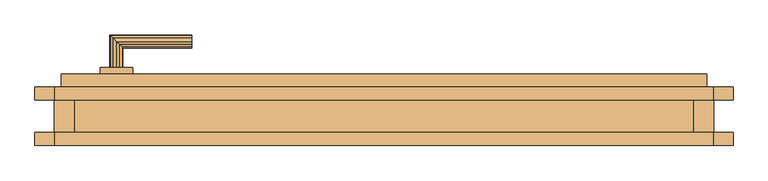
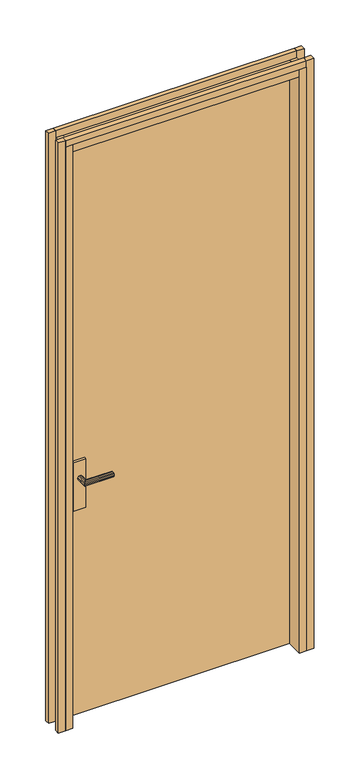
"""IFC4 building model written with IfcOpenShell, lengths in millimetres: door geometry, Tür."""

import ifcopenshell
import ifcopenshell.guid

model = None  # the IFC model being written
_history = None  # IfcOwnerHistory: only IFC2X3 demands one
_inside = {}  # id of a spatial element -> (the spatial element, [elements in it])
_under = {}  # id of a project, library or spatial element -> (it, [spatial elements below it])
_declared = {}  # id of a project -> (the project, [libraries it declares])
_typed = {}  # id of a type object -> (the type object, [elements of that type])
_made_of = {}  # id of a material, layer set ... -> (it, [elements and type objects made of it])


def new_model(schema):
    """Start an empty IFC model of exactly this schema.

    Asked for "IFC4X3", IfcOpenShell would pick the latest addendum, in which some entities
    have other attributes; the version numbers below select the first issue.
    IFC2X3 requires an IfcOwnerHistory on every rooted entity: one is made here for all.
    """
    global model, _history
    if schema == "IFC4X3":
        model = ifcopenshell.file(schema_version=(4, 3, 0, 0))
    else:
        model = ifcopenshell.file(schema=schema)
    _inside.clear()
    _under.clear()
    _declared.clear()
    _typed.clear()
    _made_of.clear()
    _history = None
    if model.schema == "IFC2X3":
        org = make("IfcOrganization", Name="unknown")
        user = make(
            "IfcPersonAndOrganization",
            ThePerson=make("IfcPerson", FamilyName="unknown"),
            TheOrganization=org,
        )
        app = make(
            "IfcApplication",
            ApplicationDeveloper=org,
            Version="unknown",
            ApplicationFullName="unknown",
            ApplicationIdentifier="unknown",
        )
        _history = make(
            "IfcOwnerHistory",
            OwningUser=user,
            OwningApplication=app,
            ChangeAction="ADDED",
            CreationDate=0,
        )
    return model


def make(cls, **values):
    """One entity of the class cls with the attributes given. An attribute that is None is left unset."""
    return model.create_entity(
        cls, **{name: value for name, value in values.items() if value is not None}
    )


def rooted(cls, **values):
    """An entity with a GlobalId (a new one), such as an element, a storey or a relation."""
    return make(cls, GlobalId=ifcopenshell.guid.new(), OwnerHistory=_history, **values)


def si_unit(unit_type, name, prefix=None):
    """IfcSIUnit, for example si_unit("LENGTHUNIT", "METRE", prefix="MILLI")."""
    return make("IfcSIUnit", UnitType=unit_type, Prefix=prefix, Name=name)


def assignment(units):
    """IfcUnitAssignment: the units of a project."""
    return None if units is None else make("IfcUnitAssignment", Units=units)


def point(xyz):
    """IfcCartesianPoint."""
    return None if xyz is None else make("IfcCartesianPoint", Coordinates=xyz)


def direction(xyz):
    """IfcDirection."""
    return None if xyz is None else make("IfcDirection", DirectionRatios=xyz)


def frame(location, z_axis=None, x_axis=None):
    """IfcAxis2Placement3D, a coordinate frame: its origin and axes. An axis left out is left unset."""
    return make(
        "IfcAxis2Placement3D",
        Location=point(location),
        Axis=direction(z_axis),
        RefDirection=direction(x_axis),
    )


def origin():
    """The frame at (0, 0, 0) with its axes left unset."""
    return frame((0.0, 0.0, 0.0))


def place(relative_to, where):
    """IfcLocalPlacement: puts the frame where relative to a parent placement (None: the world)."""
    return make(
        "IfcLocalPlacement", PlacementRelTo=relative_to, RelativePlacement=where
    )


def context(
    kind, dimensions, precision=None, world=None, true_north=None, identifier=None
):
    """IfcGeometricRepresentationContext, for example the 3D "Model" context."""
    return make(
        "IfcGeometricRepresentationContext",
        ContextIdentifier=identifier,
        ContextType=kind,
        CoordinateSpaceDimension=dimensions,
        Precision=precision,
        WorldCoordinateSystem=world,
        TrueNorth=true_north,
    )


def project(units=None, contexts=None):
    """IfcProject with its units and contexts."""
    return rooted(
        "IfcProject",
        Name="project",
        RepresentationContexts=contexts,
        UnitsInContext=assignment(units),
    )


def spatial(cls, under=None, at=None, **own):
    """A site, building, storey or space (cls), placed at a placement, below another one or the project."""
    s = rooted(cls, ObjectPlacement=at, **own)
    if under is not None:
        _under.setdefault(under.id(), (under, []))[1].append(s)
    return s


def polyline(points):
    """IfcPolyline through the points."""
    return make("IfcPolyline", Points=[point(p) for p in points])


def outline(outer, holes=None, kind="AREA"):
    """IfcArbitraryClosedProfileDef: a profile drawn as a closed curve; with holes, ...WithVoids."""
    if holes is None:
        return make("IfcArbitraryClosedProfileDef", ProfileType=kind, OuterCurve=outer)
    return make(
        "IfcArbitraryProfileDefWithVoids",
        ProfileType=kind,
        OuterCurve=outer,
        InnerCurves=holes,
    )


def extrude(swept, where, along, depth):
    """IfcExtrudedAreaSolid: the profile swept, set in the frame where, extruded along a direction by depth."""
    return make(
        "IfcExtrudedAreaSolid",
        SweptArea=swept,
        Position=where,
        ExtrudedDirection=direction(along),
        Depth=depth,
    )


def faces_of(points, faces, orient=None, outer=None):
    """IfcFace entities. A face is a list of loops; a loop is a list of indices into points, from 0.

    orient and outer hold one flag for each loop. By default every Orientation is true, the
    first loop of a face is its IfcFaceOuterBound and the others are IfcFaceBound.
    """
    made = []
    for i, loops in enumerate(faces):
        bounds = []
        for j, loop in enumerate(loops):
            is_outer = j == 0 if outer is None else outer[i][j]
            bounds.append(
                make(
                    "IfcFaceOuterBound" if is_outer else "IfcFaceBound",
                    Bound=make("IfcPolyLoop", Polygon=[points[k] for k in loop]),
                    Orientation=True if orient is None else orient[i][j],
                )
            )
        made.append(make("IfcFace", Bounds=bounds))
    return made


def faceted_brep(points, faces, orient=None, outer=None, voids=None):
    """IfcFacetedBrep: a solid bounded by flat faces; with voids (closed shells), ...WithVoids."""
    shared = [point(p) for p in points]
    hull = make("IfcClosedShell", CfsFaces=faces_of(shared, faces, orient, outer))
    if voids is None:
        return make("IfcFacetedBrep", Outer=hull)
    return make(
        "IfcFacetedBrepWithVoids",
        Outer=hull,
        Voids=[
            make(cls, CfsFaces=faces_of(shared, fs, o, b)) for cls, fs, o, b in voids
        ],
    )


def shape(context_of_items, identifier, shape_type, items):
    """IfcShapeRepresentation: the items that make up one representation, for example the "Body"."""
    return make(
        "IfcShapeRepresentation",
        ContextOfItems=context_of_items,
        RepresentationIdentifier=identifier,
        RepresentationType=shape_type,
        Items=items,
    )


def source(mapping_origin, context_of_items, identifier, shape_type, items):
    """IfcRepresentationMap: a shape defined once, which mapped items show again and again."""
    return make(
        "IfcRepresentationMap",
        MappingOrigin=mapping_origin,
        MappedRepresentation=shape(context_of_items, identifier, shape_type, items),
    )


def transform(
    local_origin,
    x_axis=None,
    y_axis=None,
    z_axis=None,
    scale=None,
    scale2=None,
    scale3=None,
    uniform=True,
):
    """IfcCartesianTransformationOperator3D, or its non-uniform kind. x_axis, y_axis, z_axis: its Axis1, 2, 3."""
    if uniform:
        return make(
            "IfcCartesianTransformationOperator3D",
            Axis1=direction(x_axis),
            Axis2=direction(y_axis),
            LocalOrigin=point(local_origin),
            Scale=scale,
            Axis3=direction(z_axis),
        )
    return make(
        "IfcCartesianTransformationOperator3DnonUniform",
        Axis1=direction(x_axis),
        Axis2=direction(y_axis),
        LocalOrigin=point(local_origin),
        Scale=scale,
        Axis3=direction(z_axis),
        Scale2=scale2,
        Scale3=scale3,
    )


def mapped(mapping_source, mapping_target):
    """IfcMappedItem: shows the shape of a source again, moved by a transform."""
    return make(
        "IfcMappedItem", MappingSource=mapping_source, MappingTarget=mapping_target
    )


def made_of(thing, what):
    """Note that an element or type object is made of a material, layer set ...; save() writes the relation."""
    if what is not None:
        _made_of.setdefault(what.id(), (what, []))[1].append(thing)
    return thing


def element(
    cls,
    number,
    at=None,
    inside=None,
    cuts=None,
    type_object=None,
    material=None,
    context=None,
    identifier="Body",
    shape_type=None,
    held_by="IfcProductDefinitionShape",
    body=None,
    shapes=None,
    **own,
):
    """One element of the class cls, such as IfcWall. Its Tag is "e" and its number.

    at: its placement. inside: the storey or other place that contains it. cuts: it is an
    opening in that element (IfcRelVoidsElement). A single representation is given by context,
    identifier, shape_type and body (its items); several are given by shapes. held_by: the class
    of the entity that holds the representations. save() writes the other relations.
    """
    e = rooted(cls, Tag="e%d" % number, ObjectPlacement=at, **own)
    if body is not None:
        shapes = [shape(context, identifier, shape_type, body)]
    if shapes is not None:
        e.Representation = make(held_by, Representations=shapes)
    if inside is not None:
        _inside.setdefault(inside.id(), (inside, []))[1].append(e)
    if cuts is not None:
        rooted(
            "IfcRelVoidsElement", RelatingBuildingElement=cuts, RelatedOpeningElement=e
        )
    if type_object is not None:
        _typed.setdefault(type_object.id(), (type_object, []))[1].append(e)
    return made_of(e, material)


def aggregate(whole, parts):
    """IfcRelAggregates: a whole, such as a stair, and the parts it consists of."""
    return rooted("IfcRelAggregates", RelatingObject=whole, RelatedObjects=parts)


def save(model, path):
    """Write the relations noted so far, then the file.

    IfcRelAggregates (storeys below a building ...), IfcRelContainedInSpatialStructure (elements
    in a storey), IfcRelDefinesByType, IfcRelAssociatesMaterial and IfcRelDeclares: one each for
    every whole, place, type object, material and project.
    """
    for whole, parts in _under.values():
        aggregate(whole, parts)
    for where, things in _inside.values():
        rooted(
            "IfcRelContainedInSpatialStructure",
            RelatedElements=things,
            RelatingStructure=where,
        )
    for kind, things in _typed.values():
        rooted("IfcRelDefinesByType", RelatedObjects=things, RelatingType=kind)
    for what, things in _made_of.values():
        rooted("IfcRelAssociatesMaterial", RelatedObjects=things, RelatingMaterial=what)
    for by, libraries in _declared.values():
        rooted("IfcRelDeclares", RelatingContext=by, RelatedDefinitions=libraries)
    model.write(path)


def door_23b21fe2(model_context):
    return source(origin(), model_context, "Body", "SolidModel", [
        faceted_brep([(100.0, 100.0, 1198.660254), (95.0, 100.0, 1200.0), (90.0, 100.0, 1198.660254), (86.339746, 100.0, 1195.0), (85.0, 100.0, 1190.0), (86.339746, 100.0, 1185.0), (90.0, 100.0, 1181.339746), (95.0, 100.0, 1180.0), (100.0, 100.0, 1181.339746), (103.660254, 100.0, 1185.0), (105.0, 100.0, 1190.0), (103.660254, 100.0, 1195.0), (95.0, 140.0, 1200.0), (90.0, 145.0, 1198.660254), (86.339746, 148.660254, 1195.0), (85.0, 150.0, 1190.0), (86.339746, 148.660254, 1185.0), (90.0, 145.0, 1181.339746), (95.0, 140.0, 1180.0), (100.0, 135.0, 1181.339746), (103.660254, 131.339746, 1185.0), (105.0, 130.0, 1190.0), (103.660254, 131.339746, 1195.0), (100.0, 135.0, 1198.660254), (210.0, 145.0, 1198.660254), (210.0, 140.0, 1200.0), (210.0, 135.0, 1198.660254), (210.0, 131.339746, 1195.0), (210.0, 130.0, 1190.0), (210.0, 131.339746, 1185.0), (210.0, 135.0, 1181.339746), (210.0, 140.0, 1180.0), (210.0, 145.0, 1181.339746), (210.0, 148.660254, 1185.0), (210.0, 150.0, 1190.0), (210.0, 148.660254, 1195.0)], [[[0, 1, 2, 3, 4, 5, 6, 7, 8, 9, 10, 11]], [[2, 1, 12, 13]], [[3, 2, 13, 14]], [[4, 3, 14, 15]], [[5, 4, 15, 16]], [[6, 5, 16, 17]], [[7, 6, 17, 18]], [[8, 7, 18, 19]], [[9, 8, 19, 20]], [[10, 9, 20, 21]], [[11, 10, 21, 22]], [[0, 11, 22, 23]], [[1, 0, 23, 12]], [[24, 25, 26, 27, 28, 29, 30, 31, 32, 33, 34, 35]], [[13, 12, 25, 24]], [[14, 13, 24, 35]], [[15, 14, 35, 34]], [[16, 15, 34, 33]], [[17, 16, 33, 32]], [[18, 17, 32, 31]], [[19, 18, 31, 30]], [[20, 19, 30, 29]], [[21, 20, 29, 28]], [[22, 21, 28, 27]], [[23, 22, 27, 26]], [[12, 23, 26, 25]]]),
        extrude(outline(polyline([(0.0, -20.0), (-30.0, -20.0), (-30.0, 0.0), (0.0, 0.0), (0.0, -20.0)])), frame((0.0, 0.0, 140.0), z_axis=(0.0, 0.0, 1.0), x_axis=(1.0, 0.0, 0.0)), (0.0, 0.0, 1.0), 2610.0),
        extrude(outline(polyline([(120.0, 90.0), (70.0, 90.0), (70.0, 100.0), (120.0, 100.0), (120.0, 90.0)])), frame((0.0, 0.0, 1050.0), z_axis=(0.0, 0.0, 1.0), x_axis=(1.0, 0.0, 0.0)), (0.0, 0.0, 1.0), 215.0),
        extrude(outline(polyline([(30.0, -20.0), (0.0, -20.0), (0.0, 70.0), (30.0, 70.0), (30.0, -20.0)])), frame((0.0, 0.0, 140.0), z_axis=(0.0, 0.0, 1.0), x_axis=(1.0, 0.0, 0.0)), (0.0, 0.0, 1.0), 2580.0),
        extrude(outline(polyline([(1010.0, -20.0), (980.0, -20.0), (980.0, 70.0), (1010.0, 70.0), (1010.0, -20.0)])), frame((0.0, 0.0, 140.0), z_axis=(0.0, 0.0, 1.0), x_axis=(1.0, 0.0, 0.0)), (0.0, 0.0, 1.0), 2580.0),
        extrude(outline(polyline([(0.0, 50.0), (-30.0, 50.0), (-30.0, 70.0), (0.0, 70.0), (0.0, 50.0)])), frame((0.0, 0.0, 140.0), z_axis=(0.0, 0.0, 1.0), x_axis=(1.0, 0.0, 0.0)), (0.0, 0.0, 1.0), 2610.0),
        extrude(outline(polyline([(1040.0, 70.0), (1040.0, 50.0), (1010.0, 50.0), (1010.0, 70.0), (1040.0, 70.0)])), frame((0.0, 0.0, 140.0), z_axis=(0.0, 0.0, 1.0), x_axis=(1.0, 0.0, 0.0)), (0.0, 0.0, 1.0), 2610.0),
        extrude(outline(polyline([(1010.0, 50.0), (0.0, 50.0), (0.0, 70.0), (1010.0, 70.0), (1010.0, 50.0)])), frame((0.0, 0.0, 2720.0), z_axis=(0.0, 0.0, 1.0), x_axis=(1.0, 0.0, 0.0)), (0.0, 0.0, 1.0), 30.0),
        extrude(outline(polyline([(1040.0, 0.0), (1040.0, -20.0), (1010.0, -20.0), (1010.0, 0.0), (1040.0, 0.0)])), frame((0.0, 0.0, 140.0), z_axis=(0.0, 0.0, 1.0), x_axis=(1.0, 0.0, 0.0)), (0.0, 0.0, 1.0), 2610.0),
        extrude(outline(polyline([(980.0, -20.0), (30.0, -20.0), (30.0, 70.0), (980.0, 70.0), (980.0, -20.0)])), frame((0.0, 0.0, 2690.0), z_axis=(0.0, 0.0, 1.0), x_axis=(1.0, 0.0, 0.0)), (0.0, 0.0, 1.0), 30.0),
        extrude(outline(polyline([(70.0, 40.0), (70.0, 50.0), (120.0, 50.0), (120.0, 40.0), (70.0, 40.0)])), frame((0.0, 0.0, 1050.0), z_axis=(0.0, 0.0, 1.0), x_axis=(1.0, 0.0, 0.0)), (0.0, 0.0, 1.0), 215.0),
        extrude(outline(polyline([(1000.0, 50.0), (10.0, 50.0), (10.0, 90.0), (1000.0, 90.0), (1000.0, 50.0)])), frame((0.0, 0.0, 140.0), z_axis=(0.0, 0.0, 1.0), x_axis=(1.0, 0.0, 0.0)), (0.0, 0.0, 1.0), 2570.0),
        extrude(outline(polyline([(1010.0, -20.0), (0.0, -20.0), (0.0, 0.0), (1010.0, 0.0), (1010.0, -20.0)])), frame((0.0, 0.0, 2720.0), z_axis=(0.0, 0.0, 1.0), x_axis=(1.0, 0.0, 0.0)), (0.0, 0.0, 1.0), 30.0),
        faceted_brep([(90.0, 40.0, 1198.660254), (95.0, 40.0, 1200.0), (100.0, 40.0, 1198.660254), (103.660254, 40.0, 1195.0), (105.0, 40.0, 1190.0), (103.660254, 40.0, 1185.0), (100.0, 40.0, 1181.339746), (95.0, 40.0, 1180.0), (90.0, 40.0, 1181.339746), (86.339746, 40.0, 1185.0), (85.0, 40.0, 1190.0), (86.339746, 40.0, 1195.0), (95.0, 0.0, 1200.0), (90.0, -5.0, 1198.660254), (86.339746, -8.660254, 1195.0), (85.0, -10.0, 1190.0), (86.339746, -8.660254, 1185.0), (90.0, -5.0, 1181.339746), (95.0, 0.0, 1180.0), (100.0, 5.0, 1181.339746), (103.660254, 8.660254, 1185.0), (105.0, 10.0, 1190.0), (103.660254, 8.660254, 1195.0), (100.0, 5.0, 1198.660254), (210.0, 5.0, 1198.660254), (210.0, 0.0, 1200.0), (210.0, -5.0, 1198.660254), (210.0, -8.660254, 1195.0), (210.0, -10.0, 1190.0), (210.0, -8.660254, 1185.0), (210.0, -5.0, 1181.339746), (210.0, 0.0, 1180.0), (210.0, 5.0, 1181.339746), (210.0, 8.660254, 1185.0), (210.0, 10.0, 1190.0), (210.0, 8.660254, 1195.0)], [[[0, 1, 2, 3, 4, 5, 6, 7, 8, 9, 10, 11]], [[12, 1, 0, 13]], [[13, 0, 11, 14]], [[14, 11, 10, 15]], [[15, 10, 9, 16]], [[16, 9, 8, 17]], [[17, 8, 7, 18]], [[18, 7, 6, 19]], [[19, 6, 5, 20]], [[20, 5, 4, 21]], [[21, 4, 3, 22]], [[22, 3, 2, 23]], [[23, 2, 1, 12]], [[24, 25, 26, 27, 28, 29, 30, 31, 32, 33, 34, 35]], [[25, 12, 13, 26]], [[26, 13, 14, 27]], [[27, 14, 15, 28]], [[28, 15, 16, 29]], [[29, 16, 17, 30]], [[30, 17, 18, 31]], [[31, 18, 19, 32]], [[32, 19, 20, 33]], [[33, 20, 21, 34]], [[34, 21, 22, 35]], [[35, 22, 23, 24]], [[24, 23, 12, 25]]]),
    ])


if __name__ == "__main__":
    model = new_model("IFC4")
    model_context = context("Model", 3, world=origin())
    ifc_project = project(units=[si_unit("LENGTHUNIT", "METRE", prefix="MILLI")], contexts=[model_context])
    site = spatial("IfcSite", under=ifc_project)
    building = spatial("IfcBuilding", under=site)
    placement = place(None, origin())
    door_shape = door_23b21fe2(model_context)
    element("IfcDoor", 1, ObjectType="Tür", at=placement, inside=building, context=model_context, shape_type="MappedRepresentation", body=[
        mapped(door_shape, transform((0.0, 0.0, 0.0), x_axis=(1.0, 0.0, 0.0), y_axis=(0.0, 1.0, 0.0), z_axis=(0.0, 0.0, 1.0))),
    ])
    save(model, "model.ifc")

# Revit data of these elements
# Type "Tür"
#   Type Mark = "53"
# Element 1 (IfcDoor, "Tür")
#   Materials on its faces: "tuer_beschlag", "tuer_holzzarge"
# Materials
#   "tuer_beschlag": class "Unassigned", colour RGB 128 128 128, transparency 0
#   "tuer_holzzarge": class "Unassigned", colour RGB 255 255 255, transparency 0
